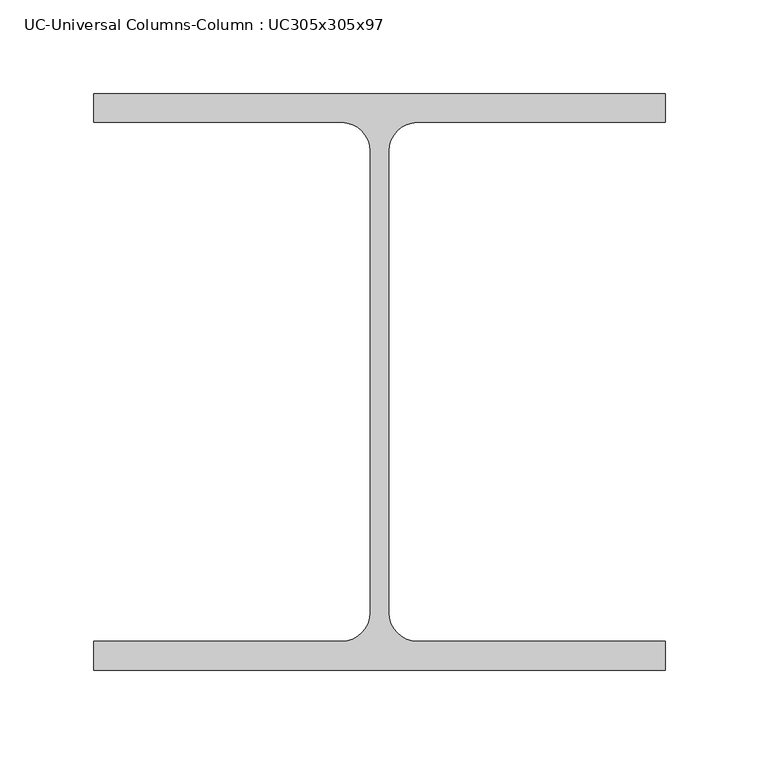
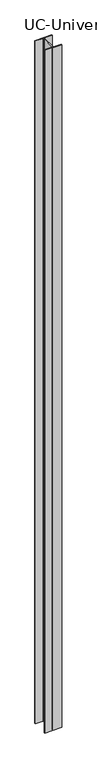
"""IFC4 building model written with IfcOpenShell, lengths in millimetres: column geometry, UC-Universal Columns-Column : UC305x305x97."""

import ifcopenshell
import ifcopenshell.guid

model = None  # the IFC model being written
_history = None  # IfcOwnerHistory: only IFC2X3 demands one
_inside = {}  # id of a spatial element -> (the spatial element, [elements in it])
_under = {}  # id of a project, library or spatial element -> (it, [spatial elements below it])
_declared = {}  # id of a project -> (the project, [libraries it declares])
_typed = {}  # id of a type object -> (the type object, [elements of that type])
_made_of = {}  # id of a material, layer set ... -> (it, [elements and type objects made of it])


def new_model(schema):
    """Start an empty IFC model of exactly this schema.

    Asked for "IFC4X3", IfcOpenShell would pick the latest addendum, in which some entities
    have other attributes; the version numbers below select the first issue.
    IFC2X3 requires an IfcOwnerHistory on every rooted entity: one is made here for all.
    """
    global model, _history
    if schema == "IFC4X3":
        model = ifcopenshell.file(schema_version=(4, 3, 0, 0))
    else:
        model = ifcopenshell.file(schema=schema)
    _inside.clear()
    _under.clear()
    _declared.clear()
    _typed.clear()
    _made_of.clear()
    _history = None
    if model.schema == "IFC2X3":
        org = make("IfcOrganization", Name="unknown")
        user = make(
            "IfcPersonAndOrganization",
            ThePerson=make("IfcPerson", FamilyName="unknown"),
            TheOrganization=org,
        )
        app = make(
            "IfcApplication",
            ApplicationDeveloper=org,
            Version="unknown",
            ApplicationFullName="unknown",
            ApplicationIdentifier="unknown",
        )
        _history = make(
            "IfcOwnerHistory",
            OwningUser=user,
            OwningApplication=app,
            ChangeAction="ADDED",
            CreationDate=0,
        )
    return model


def make(cls, **values):
    """One entity of the class cls with the attributes given. An attribute that is None is left unset."""
    return model.create_entity(
        cls, **{name: value for name, value in values.items() if value is not None}
    )


def rooted(cls, **values):
    """An entity with a GlobalId (a new one), such as an element, a storey or a relation."""
    return make(cls, GlobalId=ifcopenshell.guid.new(), OwnerHistory=_history, **values)


def si_unit(unit_type, name, prefix=None):
    """IfcSIUnit, for example si_unit("LENGTHUNIT", "METRE", prefix="MILLI")."""
    return make("IfcSIUnit", UnitType=unit_type, Prefix=prefix, Name=name)


def assignment(units):
    """IfcUnitAssignment: the units of a project."""
    return None if units is None else make("IfcUnitAssignment", Units=units)


def point(xyz):
    """IfcCartesianPoint."""
    return None if xyz is None else make("IfcCartesianPoint", Coordinates=xyz)


def direction(xyz):
    """IfcDirection."""
    return None if xyz is None else make("IfcDirection", DirectionRatios=xyz)


def frame(location, z_axis=None, x_axis=None):
    """IfcAxis2Placement3D, a coordinate frame: its origin and axes. An axis left out is left unset."""
    return make(
        "IfcAxis2Placement3D",
        Location=point(location),
        Axis=direction(z_axis),
        RefDirection=direction(x_axis),
    )


def frame_2d(location, x_axis=None):
    """IfcAxis2Placement2D, a coordinate frame in the plane: its origin and x axis."""
    return make(
        "IfcAxis2Placement2D", Location=point(location), RefDirection=direction(x_axis)
    )


def origin():
    """The frame at (0, 0, 0) with its axes left unset."""
    return frame((0.0, 0.0, 0.0))


def place(relative_to, where):
    """IfcLocalPlacement: puts the frame where relative to a parent placement (None: the world)."""
    return make(
        "IfcLocalPlacement", PlacementRelTo=relative_to, RelativePlacement=where
    )


def context(
    kind, dimensions, precision=None, world=None, true_north=None, identifier=None
):
    """IfcGeometricRepresentationContext, for example the 3D "Model" context."""
    return make(
        "IfcGeometricRepresentationContext",
        ContextIdentifier=identifier,
        ContextType=kind,
        CoordinateSpaceDimension=dimensions,
        Precision=precision,
        WorldCoordinateSystem=world,
        TrueNorth=true_north,
    )


def project(units=None, contexts=None):
    """IfcProject with its units and contexts."""
    return rooted(
        "IfcProject",
        Name="project",
        RepresentationContexts=contexts,
        UnitsInContext=assignment(units),
    )


def spatial(cls, under=None, at=None, **own):
    """A site, building, storey or space (cls), placed at a placement, below another one or the project."""
    s = rooted(cls, ObjectPlacement=at, **own)
    if under is not None:
        _under.setdefault(under.id(), (under, []))[1].append(s)
    return s


def polyline(points):
    """IfcPolyline through the points."""
    return make("IfcPolyline", Points=[point(p) for p in points])


def circle_curve(where, radius):
    """IfcCircle in the frame where."""
    return make("IfcCircle", Position=where, Radius=radius)


def trimmed(basis, trim1, trim2, sense, master):
    """IfcTrimmedCurve: the piece of a basis curve between two trims."""
    return make(
        "IfcTrimmedCurve",
        BasisCurve=basis,
        Trim1=trim1,
        Trim2=trim2,
        SenseAgreement=sense,
        MasterRepresentation=master,
    )


def segment(curve, same_sense, transition):
    """IfcCompositeCurveSegment."""
    return make(
        "IfcCompositeCurveSegment",
        Transition=transition,
        SameSense=same_sense,
        ParentCurve=curve,
    )


def composite_curve(segments, self_intersect=None):
    """IfcCompositeCurve: segments joined end to end."""
    return make("IfcCompositeCurve", Segments=segments, SelfIntersect=self_intersect)


def outline(outer, holes=None, kind="AREA"):
    """IfcArbitraryClosedProfileDef: a profile drawn as a closed curve; with holes, ...WithVoids."""
    if holes is None:
        return make("IfcArbitraryClosedProfileDef", ProfileType=kind, OuterCurve=outer)
    return make(
        "IfcArbitraryProfileDefWithVoids",
        ProfileType=kind,
        OuterCurve=outer,
        InnerCurves=holes,
    )


def extrude(swept, where, along, depth):
    """IfcExtrudedAreaSolid: the profile swept, set in the frame where, extruded along a direction by depth."""
    return make(
        "IfcExtrudedAreaSolid",
        SweptArea=swept,
        Position=where,
        ExtrudedDirection=direction(along),
        Depth=depth,
    )


def shape(context_of_items, identifier, shape_type, items):
    """IfcShapeRepresentation: the items that make up one representation, for example the "Body"."""
    return make(
        "IfcShapeRepresentation",
        ContextOfItems=context_of_items,
        RepresentationIdentifier=identifier,
        RepresentationType=shape_type,
        Items=items,
    )


def source(mapping_origin, context_of_items, identifier, shape_type, items):
    """IfcRepresentationMap: a shape defined once, which mapped items show again and again."""
    return make(
        "IfcRepresentationMap",
        MappingOrigin=mapping_origin,
        MappedRepresentation=shape(context_of_items, identifier, shape_type, items),
    )


def transform(
    local_origin,
    x_axis=None,
    y_axis=None,
    z_axis=None,
    scale=None,
    scale2=None,
    scale3=None,
    uniform=True,
):
    """IfcCartesianTransformationOperator3D, or its non-uniform kind. x_axis, y_axis, z_axis: its Axis1, 2, 3."""
    if uniform:
        return make(
            "IfcCartesianTransformationOperator3D",
            Axis1=direction(x_axis),
            Axis2=direction(y_axis),
            LocalOrigin=point(local_origin),
            Scale=scale,
            Axis3=direction(z_axis),
        )
    return make(
        "IfcCartesianTransformationOperator3DnonUniform",
        Axis1=direction(x_axis),
        Axis2=direction(y_axis),
        LocalOrigin=point(local_origin),
        Scale=scale,
        Axis3=direction(z_axis),
        Scale2=scale2,
        Scale3=scale3,
    )


def mapped(mapping_source, mapping_target):
    """IfcMappedItem: shows the shape of a source again, moved by a transform."""
    return make(
        "IfcMappedItem", MappingSource=mapping_source, MappingTarget=mapping_target
    )


def made_of(thing, what):
    """Note that an element or type object is made of a material, layer set ...; save() writes the relation."""
    if what is not None:
        _made_of.setdefault(what.id(), (what, []))[1].append(thing)
    return thing


def element(
    cls,
    number,
    at=None,
    inside=None,
    cuts=None,
    type_object=None,
    material=None,
    context=None,
    identifier="Body",
    shape_type=None,
    held_by="IfcProductDefinitionShape",
    body=None,
    shapes=None,
    **own,
):
    """One element of the class cls, such as IfcWall. Its Tag is "e" and its number.

    at: its placement. inside: the storey or other place that contains it. cuts: it is an
    opening in that element (IfcRelVoidsElement). A single representation is given by context,
    identifier, shape_type and body (its items); several are given by shapes. held_by: the class
    of the entity that holds the representations. save() writes the other relations.
    """
    e = rooted(cls, Tag="e%d" % number, ObjectPlacement=at, **own)
    if body is not None:
        shapes = [shape(context, identifier, shape_type, body)]
    if shapes is not None:
        e.Representation = make(held_by, Representations=shapes)
    if inside is not None:
        _inside.setdefault(inside.id(), (inside, []))[1].append(e)
    if cuts is not None:
        rooted(
            "IfcRelVoidsElement", RelatingBuildingElement=cuts, RelatedOpeningElement=e
        )
    if type_object is not None:
        _typed.setdefault(type_object.id(), (type_object, []))[1].append(e)
    return made_of(e, material)


def aggregate(whole, parts):
    """IfcRelAggregates: a whole, such as a stair, and the parts it consists of."""
    return rooted("IfcRelAggregates", RelatingObject=whole, RelatedObjects=parts)


def save(model, path):
    """Write the relations noted so far, then the file.

    IfcRelAggregates (storeys below a building ...), IfcRelContainedInSpatialStructure (elements
    in a storey), IfcRelDefinesByType, IfcRelAssociatesMaterial and IfcRelDeclares: one each for
    every whole, place, type object, material and project.
    """
    for whole, parts in _under.values():
        aggregate(whole, parts)
    for where, things in _inside.values():
        rooted(
            "IfcRelContainedInSpatialStructure",
            RelatedElements=things,
            RelatingStructure=where,
        )
    for kind, things in _typed.values():
        rooted("IfcRelDefinesByType", RelatedObjects=things, RelatingType=kind)
    for what, things in _made_of.values():
        rooted("IfcRelAssociatesMaterial", RelatedObjects=things, RelatingMaterial=what)
    for by, libraries in _declared.values():
        rooted("IfcRelDeclares", RelatingContext=by, RelatedDefinitions=libraries)
    model.write(path)


def uc_universal_columns_column_uc305x305x97_fcd1f718(model_context):
    return source(origin(), model_context, "Body", "SweptSolid", [
        extrude(outline(composite_curve([segment(polyline([(152.65, 153.95), (152.65, 138.55), (20.15, 138.55)]), True, "CONTINUOUS"), segment(trimmed(circle_curve(frame_2d((20.15, 123.35)), 15.2), [point((20.15, 138.55))], [point((4.95, 123.35))], True, "CARTESIAN"), True, "CONTINUOUS"), segment(polyline([(4.95, 123.35), (4.95, -123.35)]), True, "CONTINUOUS"), segment(trimmed(circle_curve(frame_2d((20.15, -123.35)), 15.2), [point((4.95, -123.35))], [point((20.15, -138.55))], True, "CARTESIAN"), True, "CONTINUOUS"), segment(polyline([(20.15, -138.55), (152.65, -138.55), (152.65, -153.95), (-152.65, -153.95), (-152.65, -138.55), (-20.15, -138.55)]), True, "CONTINUOUS"), segment(trimmed(circle_curve(frame_2d((-20.15, -123.35)), 15.2), [point((-20.15, -138.55))], [point((-4.95, -123.35))], True, "CARTESIAN"), True, "CONTINUOUS"), segment(polyline([(-4.95, -123.35), (-4.95, 123.35)]), True, "CONTINUOUS"), segment(trimmed(circle_curve(frame_2d((-20.15, 123.35)), 15.2), [point((-4.95, 123.35))], [point((-20.15, 138.55))], True, "CARTESIAN"), True, "CONTINUOUS"), segment(polyline([(-20.15, 138.55), (-152.65, 138.55), (-152.65, 153.95), (152.65, 153.95)]), True, "CONTINUOUS")], self_intersect=False)), frame((0.0, 0.0, -594.0), z_axis=(0.0, 0.0, 1.0), x_axis=(1.0, 0.0, 0.0)), (0.0, 0.0, 1.0), 13033.0),
    ])


if __name__ == "__main__":
    model = new_model("IFC4")
    model_context = context("Model", 3, world=origin())
    ifc_project = project(units=[si_unit("LENGTHUNIT", "METRE", prefix="MILLI")], contexts=[model_context])
    site = spatial("IfcSite", under=ifc_project)
    building = spatial("IfcBuilding", under=site)
    placement = place(None, origin())
    uc_universal_columns_column_uc305x305x97_shape = uc_universal_columns_column_uc305x305x97_fcd1f718(model_context)
    element("IfcColumn", 1, ObjectType="UC-Universal Columns-Column : UC305x305x97", at=placement, inside=building, context=model_context, shape_type="MappedRepresentation", body=[
        mapped(uc_universal_columns_column_uc305x305x97_shape, transform((0.0, 0.0, 0.0), x_axis=(1.0, 0.0, 0.0), y_axis=(0.0, 1.0, 0.0), z_axis=(0.0, 0.0, 1.0))),
    ])
    save(model, "model.ifc")

# Revit data of these elements
# Type "UC-Universal Columns-Column : UC305x305x97"
#   Section Name Key = "UC305x305x97"
#   Cost = 2
#   Width = 30.53 cm
#   Web Thickness = 0.99 cm
#   Web Fillet = 1.52 cm
#   Warping Constant = 1560000.0 cm⁶
#   Torsional Moment of Inertia = 91.20 cm⁴
#   Section Area = 123.0 cm²
#   Plastic Modulus weak axis = 726.0 cm³
#   Plastic Modulus strong axis = 1592.0 cm³
#   Nominal Weight = 96.8996 kgf/m
#   Moment of Inertia weak axis = 7308.00 cm⁴
#   Moment of Inertia strong axis = 22249.00 cm⁴
#   Height = 30.79 cm
#   Flange Thickness = 1.54 cm
#   Elastic Modulus weak axis = 479.0 cm³
#   Elastic Modulus strong axis = 1445.0 cm³
#   Centroid Vertical = 15.395 cm
#   Centroid Horizontal = 15.265 cm
#   Bolt Spacing = 14.0 cm
#   Structural Material [instance default] = Metal - Steel 43-275
#   Type Comments = ""
#   Assembly Code = ""
# Element 1 (IfcColumn, "UC-Universal Columns-Column : UC305x305x97")
#   Materials on its faces: "Metal - Steel 43-275"
# Materials
#   "Metal - Steel 43-275": class "Metal", colour RGB 247 247 247, transparency 0, Cost = 0
